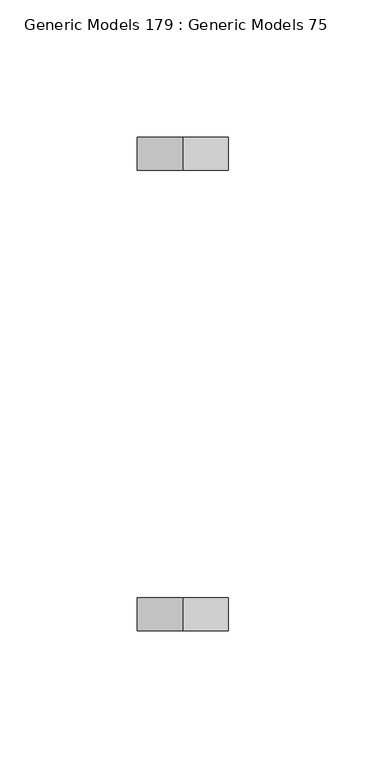
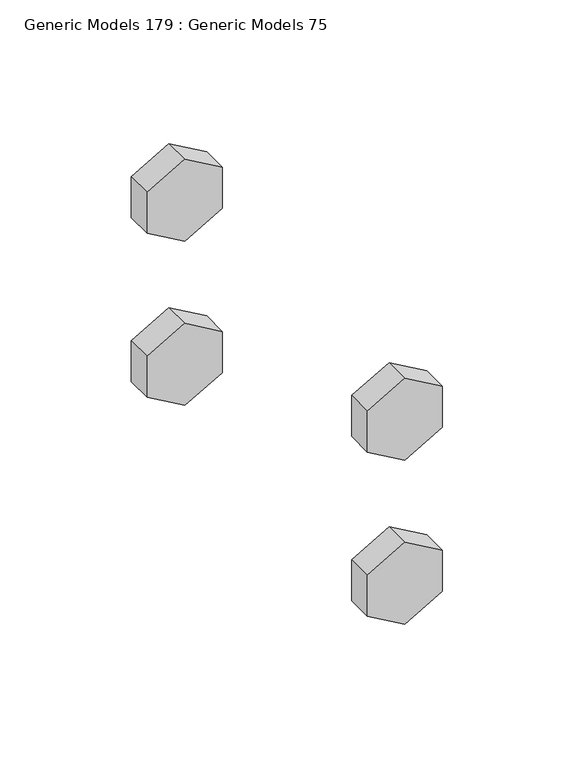
"""IFC4 building model written with IfcOpenShell, lengths in millimetres: proxy geometry, Generic Models 179 : Generic Models 75."""

from ifc_helpers import new_model, si_unit, frame, origin, place, context, project, spatial, polyline, outline, extrude, source, transform, mapped, element, save


def generic_models_179_generic_models_75_3dcc9f73(model_context):
    return source(origin(), model_context, "Body", "SweptSolid", [
        extrude(outline(polyline([(271832.3875, 31991.9073871), (271851.4375, 31991.9073871), (271860.9625, 31975.4096032), (271851.4375, 31958.9118192), (271832.3875, 31958.9118192), (271822.8625, 31975.4096032), (271832.3875, 31991.9073871)])), frame((0.0, 36485.2082942, 0.0), z_axis=(0.0, 1.0, 0.0), x_axis=(0.0, 0.0, 1.0)), (0.0, 0.0, 1.0), 11.90625),
        extrude(outline(polyline([(271756.1875, 31991.9073871), (271775.2375, 31991.9073871), (271784.7625, 31975.4096032), (271775.2375, 31958.9118192), (271756.1875, 31958.9118192), (271746.6625, 31975.4096032), (271756.1875, 31991.9073871)])), frame((0.0, 36485.2082942, 0.0), z_axis=(0.0, 1.0, 0.0), x_axis=(0.0, 0.0, 1.0)), (0.0, 0.0, 1.0), 11.90625),
        extrude(outline(polyline([(271832.3875, 31991.9073871), (271851.4375, 31991.9073871), (271860.9625, 31975.4096032), (271851.4375, 31958.9118192), (271832.3875, 31958.9118192), (271822.8625, 31975.4096032), (271832.3875, 31991.9073871)])), frame((0.0, 36317.7270442, 0.0), z_axis=(0.0, 1.0, 0.0), x_axis=(0.0, 0.0, 1.0)), (0.0, 0.0, 1.0), 11.90625),
        extrude(outline(polyline([(271756.1875, 31991.9073871), (271775.2375, 31991.9073871), (271784.7625, 31975.4096032), (271775.2375, 31958.9118192), (271756.1875, 31958.9118192), (271746.6625, 31975.4096032), (271756.1875, 31991.9073871)])), frame((0.0, 36317.7270442, 0.0), z_axis=(0.0, 1.0, 0.0), x_axis=(0.0, 0.0, 1.0)), (0.0, 0.0, 1.0), 11.90625),
    ])


if __name__ == "__main__":
    model = new_model("IFC4")
    model_context = context("Model", 3, world=origin())
    ifc_project = project(units=[si_unit("LENGTHUNIT", "METRE", prefix="MILLI")], contexts=[model_context])
    site = spatial("IfcSite", under=ifc_project)
    building = spatial("IfcBuilding", under=site)
    placement = place(None, origin())
    generic_models_179_generic_models_75_shape = generic_models_179_generic_models_75_3dcc9f73(model_context)
    element("IfcBuildingElementProxy", 1, Name="Generic Models 179 : Generic Models 75", ObjectType="Generic Models 179 : Generic Models 75", at=placement, inside=building, context=model_context, shape_type="MappedRepresentation", body=[
        mapped(generic_models_179_generic_models_75_shape, transform((0.0, 0.0, 0.0), x_axis=(1.0, 0.0, 0.0), y_axis=(0.0, 1.0, 0.0), z_axis=(0.0, 0.0, 1.0))),
    ])
    save(model, "model.ifc")
